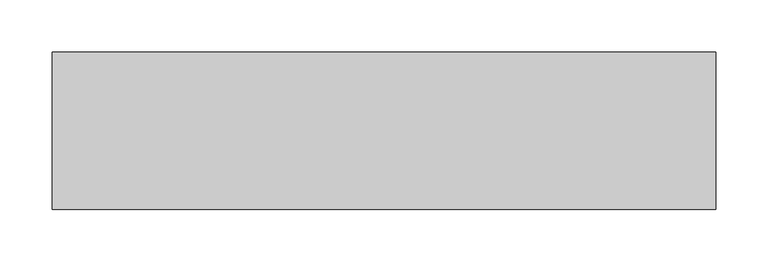
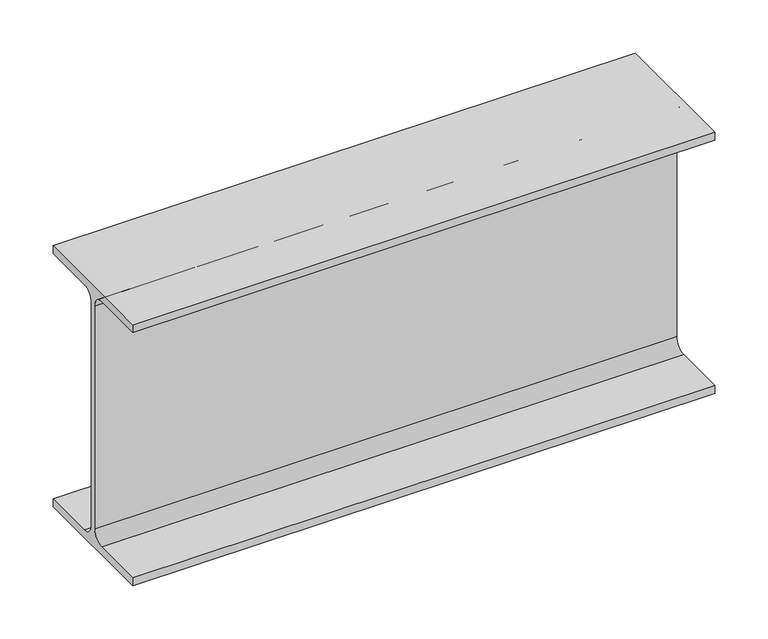
"""IFC4 building model written with IfcOpenShell, lengths in millimetres: beam geometry, 0912_Steel Framing_H-KSD3502 : H_SB_ASB_H-300x150x6.5x9."""

from ifc_helpers import new_model, si_unit, point, frame, frame_2d, origin, place, context, project, spatial, polyline, circle_curve, trimmed, segment, composite_curve, outline, extrude, source, transform, mapped, element, save


def beam_a0ee07d4(model_context):
    return source(origin(), model_context, "Body", "SweptSolid", [
        extrude(outline(composite_curve([segment(polyline([(75.0, -141.0), (75.0, -150.0), (-75.0, -150.0), (-75.0, -141.0), (-16.25, -141.0)]), True, "CONTINUOUS"), segment(trimmed(circle_curve(frame_2d((-16.25, -128.0)), 13.0), [point((-16.25, -141.0))], [point((-3.25, -128.0))], True, "CARTESIAN"), True, "CONTINUOUS"), segment(polyline([(-3.25, -128.0), (-3.25, 128.0)]), True, "CONTINUOUS"), segment(trimmed(circle_curve(frame_2d((-16.25, 128.0)), 13.0), [point((-3.25, 128.0))], [point((-16.25, 141.0))], True, "CARTESIAN"), True, "CONTINUOUS"), segment(polyline([(-16.25, 141.0), (-75.0, 141.0), (-75.0, 150.0), (75.0, 150.0), (75.0, 141.0), (16.25, 141.0)]), True, "CONTINUOUS"), segment(trimmed(circle_curve(frame_2d((16.25, 128.0)), 13.0), [point((16.25, 141.0))], [point((3.25, 128.0))], True, "CARTESIAN"), True, "CONTINUOUS"), segment(polyline([(3.25, 128.0), (3.25, -128.0)]), True, "CONTINUOUS"), segment(trimmed(circle_curve(frame_2d((16.25, -128.0)), 13.0), [point((3.25, -128.0))], [point((16.25, -141.0))], True, "CARTESIAN"), True, "CONTINUOUS"), segment(polyline([(16.25, -141.0), (75.0, -141.0)]), True, "CONTINUOUS")], self_intersect=False)), frame((-349.8, 0.0, 0.0), z_axis=(1.0, 0.0, 0.0), x_axis=(0.0, 1.0, 0.0)), (0.0, 0.0, 1.0), 632.1),
    ])


if __name__ == "__main__":
    model = new_model("IFC4")
    model_context = context("Model", 3, world=origin())
    ifc_project = project(units=[si_unit("LENGTHUNIT", "METRE", prefix="MILLI")], contexts=[model_context])
    site = spatial("IfcSite", under=ifc_project)
    building = spatial("IfcBuilding", under=site)
    placement = place(None, origin())
    beam_shape = beam_a0ee07d4(model_context)
    element("IfcBeam", 1, ObjectType="0912_Steel Framing_H-KSD3502 : H_SB_ASB_H-300x150x6.5x9", at=placement, inside=building, context=model_context, shape_type="MappedRepresentation", body=[
        mapped(beam_shape, transform((0.0, 0.0, 0.0), x_axis=(1.0, 0.0, 0.0), y_axis=(0.0, 1.0, 0.0), z_axis=(0.0, 0.0, 1.0))),
    ])
    save(model, "model.ifc")

# Revit data of these elements
# Type "0912_Steel Framing_H-KSD3502 : H_SB_ASB_H-300x150x6.5x9"
#   H_WM Code_1 = "S01AA002-00001 | Main Steel Structure Fabrication Work | Shelter/Building | Medium Steel - Standard (90KG/M>Weight≥30KG/M) | Material: (   )"
#   H_WM Code_2 = "S03AA028-00001 | Main Steel Structure Erection Work | Shelter/Building | Medium Steel (90KG/M>Weight≥30KG/M) | Material: (   )"
#   H_WM Code_3 = "S01AA010-00001 | Main Steel Structure Fabrication Work | Shelter/Building | Steel Painting/Coating | for Non-Fireproofed Steel Surface, Surface Preparation, Primer, Second & Final Coat | Material: (   )"
#   H_Q'ty Cal Type Tag = "SB-Q2"
#   Width = 15.0 cm
#   Web Thickness = 0.65 cm
#   Web Fillet = 1.3 cm
#   Warping Constant = 107000.0 cm⁶
#   W = 0
#   Torsional Moment of Inertia = 9.9539 cm⁴
#   Section Area = 46.78 cm²
#   Plastic Modulus weak axis = 105.0 cm³
#   Plastic Modulus strong axis = 542.0 cm³
#   Perimeter = 1.17 m²/m
#   Nominal Weight = 36.70 kgf/m
#   Moment of Inertia weak axis = 508.00 cm⁴
#   Moment of Inertia strong axis = 7210.00 cm⁴
#   Height = 30.0 cm
#   Flange Thickness = 0.9 cm
#   Elastic Modulus weak axis = 67.7 cm³
#   Elastic Modulus strong axis = 481.0 cm³
#   Centroid Vertical = 15.0 cm
#   Centroid Horizontal = 7.5 cm
#   Ix = 72100000
#   Length [instance default] = 1.5240 m
#   Zx = 542000
#   b = 0.1500 m
#   h = 0.3000 m
#   r = 0.0130 m
#   s = 0.0065 m
#   t = 0.0090 m
#   A = 0.004678 m²
#   Structural Material [instance default] = Steel, 45-345
#   Assembly Code = ""
# Element 1 (IfcBeam, "0912_Steel Framing_H-KSD3502 : H_SB_ASB_H-300x150x6.5x9")
#   Structural Material = none
# Materials
#   "Steel, 45-345": class "Metal", colour RGB 189 187 185, transparency 0, Description = "Steel 345 MPa", Cost = 0
